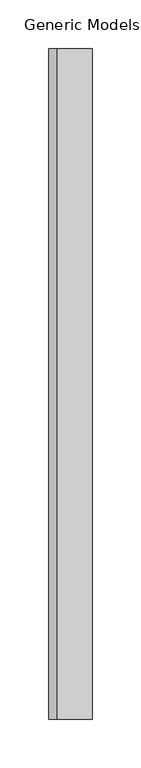
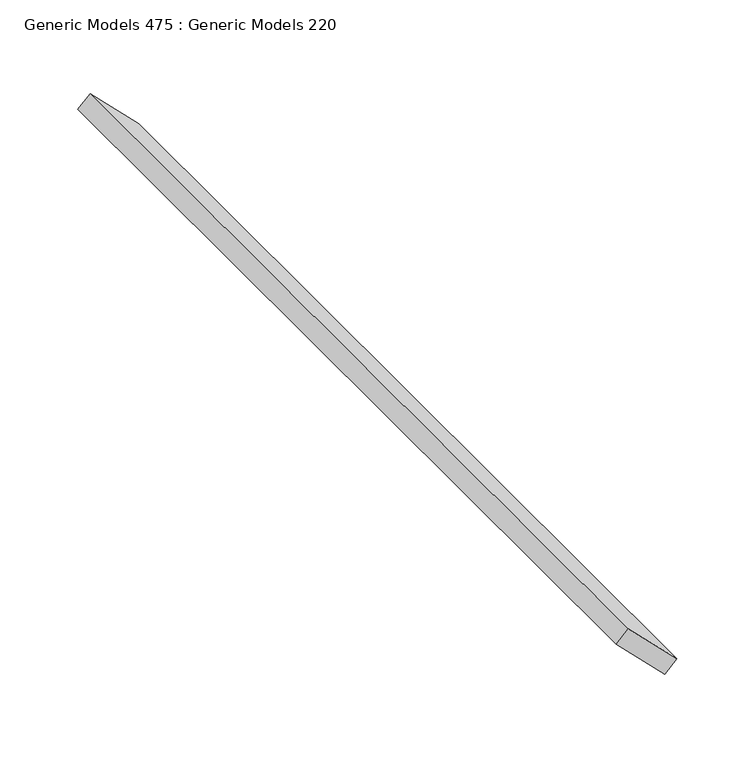
"""IFC4 building model written with IfcOpenShell, lengths in millimetres: proxy geometry, Generic Models 475 : Generic Models 220."""

from ifc_helpers import new_model, si_unit, frame, origin, place, context, project, spatial, polyline, outline, extrude, source, transform, mapped, element, save


def generic_models_475_generic_models_220_28df3cce(model_context):
    return source(origin(), model_context, "Body", "SweptSolid", [
        extrude(outline(polyline([(0.0, -50.8), (0.0, 0.0), (690.8142348, 0.0), (690.8142348, -50.8), (0.0, -50.8)])), frame((-6899.085451, -4564.8872686, 128005.6762561), z_axis=(0.7071067811865582, 0.0, 0.7071067811865369), x_axis=(0.0, 1.0, 0.0)), (0.0, 0.0, 1.0), 12.7),
    ])


if __name__ == "__main__":
    model = new_model("IFC4")
    model_context = context("Model", 3, world=origin())
    ifc_project = project(units=[si_unit("LENGTHUNIT", "METRE", prefix="MILLI")], contexts=[model_context])
    site = spatial("IfcSite", under=ifc_project)
    building = spatial("IfcBuilding", under=site)
    placement = place(None, origin())
    generic_models_475_generic_models_220_shape = generic_models_475_generic_models_220_28df3cce(model_context)
    element("IfcBuildingElementProxy", 1, Name="Generic Models 475 : Generic Models 220", ObjectType="Generic Models 475 : Generic Models 220", at=placement, inside=building, context=model_context, shape_type="MappedRepresentation", body=[
        mapped(generic_models_475_generic_models_220_shape, transform((0.0, 0.0, 0.0), x_axis=(1.0, 0.0, 0.0), y_axis=(0.0, 1.0, 0.0), z_axis=(0.0, 0.0, 1.0))),
    ])
    save(model, "model.ifc")

# Revit data of these elements
# Element 1 (IfcBuildingElementProxy, "Generic Models 475 : Generic Models 220")
#   Materials on its faces: "_WOOD TONE ALUMINUM EXTRUSION SLAT BY KNOTWOOD"
# Materials
#   "_WOOD TONE ALUMINUM EXTRUSION SLAT BY KNOTWOOD": class "Generic", colour RGB 177 130 114, transparency 0, Cost = 0
